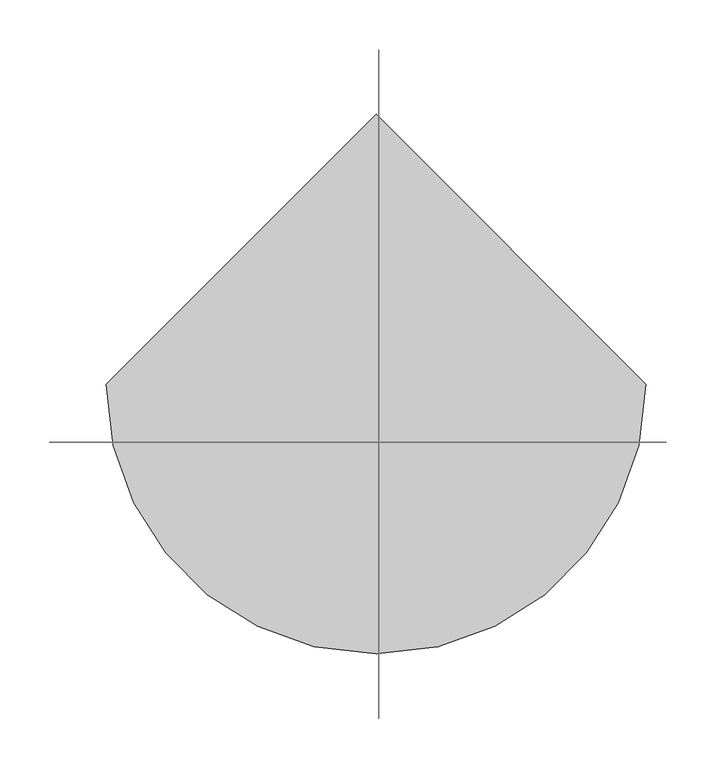
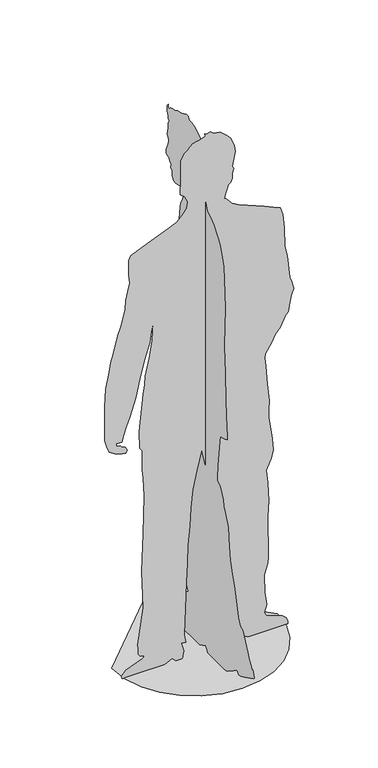
"""IFC4 building model written with IfcOpenShell, lengths in millimetres: proxy geometry, brennan 23759 : brennan 23759."""

from ifc_helpers import new_model, si_unit, origin, place, context, project, spatial, triangles, source, transform, mapped, element, save


def entourage_5001038d(model_context):
    return source(origin(), model_context, "Body", "Tessellation", [
        triangles([(-272.8237541, 0.0, 0.0), (-265.6179985, -62.508739, 0.0), (-245.0759747, -119.914065, 0.0), (-212.8506706, -170.5790321, 0.0), (-170.5790321, -212.8506706, 0.0), (-119.914065, -245.0759747, 0.0), (-62.508739, -265.6179985, 0.0), (0.0, -272.8237541, 0.0), (62.508739, -265.6179985, 0.0), (119.914065, -245.0759747, 0.0), (170.5790321, -212.8506706, 0.0), (212.8506706, -170.5790321, 0.0), (245.0759747, -119.914065, 0.0), (265.6179985, -62.508739, 0.0), (272.8237541, 0.0, 0.0), (0.0, 272.8237541, 0.0), (17.3323325, -58.9941234, 1803.4452976), (28.5662524, -58.9941234, 1794.2976002), (51.3711104, -58.9941234, 1790.7991219), (70.6934502, -58.9941234, 1773.5309898), (84.1902009, -58.9941234, 1758.6380035), (96.7561399, -58.9941234, 1728.4508926), (100.5435813, -58.9941234, 1706.8495949), (90.8824069, -58.9941234, 1658.3351143), (94.6698392, -58.9941234, 1649.7491558), (90.8824069, -58.9941234, 1634.1179878), (91.1873301, -58.9941234, 1616.5128124), (85.8271467, -58.9941234, 1604.5888309), (77.5300878, -58.9941234, 1597.8966522), (73.501927, -58.9941234, 1586.9836555), (68.8960218, -58.9941234, 1573.3586151), (64.8036662, -58.9941234, 1555.3682888), (71.4316773, -58.9941234, 1551.0351231), (89.1331223, -58.9941234, 1530.3004875), (111.1516093, -58.9941234, 1515.9371201), (196.7219676, -58.9941234, 1481.0959328), (225.657338, -58.9941234, 1468.1127136), (247.9325954, -58.9941234, 1457.5047855), (256.0691627, -58.9941234, 1432.3247818), (262.215717, -58.9941234, 1382.7991711), (262.66509, -58.9941234, 1321.2533638), (271.5880192, -58.9941234, 1282.6247623), (279.4517653, -58.9941234, 1205.6402899), (284.9242873, -58.9941234, 1193.4594927), (293.4941676, -58.9941234, 1162.1650366), (284.2181531, -58.9941234, 1141.3180532), (280.6072543, -58.9941234, 1114.9985842), (275.7927226, -58.9941234, 1086.5607124), (264.7353307, -58.9941234, 1075.5033205), (249.1201864, -58.9941234, 1041.994174), (232.4458408, -58.9941234, 1023.1532455), (220.2169179, -58.9941234, 999.2892225), (205.9658801, -58.9941234, 976.5806522), (198.7601244, -58.9941234, 964.9294739), (196.7701296, -58.9941234, 951.8820871), (200.0600633, -58.9941234, 923.7972462), (205.0190266, -58.9941234, 860.4700796), (212.3050281, -58.9941234, 798.3625334), (211.149539, -58.9941234, 769.7963264), (210.4273629, -58.9941234, 741.8559534), (222.8488612, -58.9941234, 662.8173185), (225.7375839, -58.9941234, 622.9850115), (219.783605, -58.9941234, 595.2853941), (202.3710232, -58.9941234, 560.3639428), (207.8917073, -58.9941234, 513.5987377), (210.2187274, -58.9941234, 450.4159664), (207.9398512, -58.9941234, 397.7288844), (208.9027466, -58.9941234, 255.6840118), (207.233717, -58.9941234, 233.2482628), (195.7751141, -58.9941234, 197.7330251), (197.8774567, -58.9941234, 134.2774325), (204.9387807, -58.9941234, 92.0539469), (196.6417399, -58.9941234, 65.5739907), (202.0179743, -58.9941234, 54.6289466), (255.0581052, -58.9941234, 33.717807), (267.6721972, -58.9941234, 23.7196187), (272.9039999, -58.9941234, 10.2549632), (273.241007, -58.9941234, 0.6900836), (261.9268538, -58.9941234, 0.0), (221.8699057, -58.9941234, 0.0), (191.6025126, -58.9941234, 0.0), (171.4616999, -58.9941234, 0.0), (142.0127888, -58.9941234, 0.0), (122.658347, -58.9941234, 10.2549632), (115.8538023, -58.9941234, 0.0), (84.7037506, -58.9941234, 0.0), (81.3977659, -58.9941234, 24.6504281), (90.4972469, -58.9941234, 46.3800406), (91.4601514, -58.9941234, 126.9111943), (80.8842163, -58.9941234, 157.4835015), (66.3122224, -58.9941234, 219.2861063), (39.8483172, -58.9941234, 475.5318026), (27.828023, -58.9941234, 536.9973822), (20.5099263, -58.9941234, 568.3079347), (16.1768435, -58.9941234, 596.7939503), (7.3020474, -58.9941234, 627.8958309), (0.1283877, -58.9941234, 657.1200645), (-6.290995, -58.9941234, 688.2861855), (-10.7524653, -58.9941234, 704.8000757), (-18.1668519, -58.9941234, 671.7563078), (-27.0095523, -58.9941234, 638.4076166), (-40.0408972, -58.9941234, 577.9049143), (-46.7170567, -58.9941234, 516.1504352), (-49.7181181, -58.9941234, 452.6627406), (-56.8436324, -58.9941234, 389.7046649), (-58.3682351, -58.9941234, 326.3132581), (-60.7113106, -58.9941234, 262.1675732), (-67.9652101, -58.9941234, 81.9755105), (-63.4555971, -58.9941234, 53.5857962), (-78.1720272, -58.9941234, 56.1374982), (-69.4416689, -58.9941234, 26.5441465), (-73.501927, -58.9941234, 0.0), (-95.0389573, -58.9941234, 0.0), (-107.8616757, -58.9941234, 13.0634434), (-134.0688061, -58.9941234, 0.0), (-208.1805705, -58.9941234, 0.0), (-272.502789, -58.9941234, 0.0), (-275.9692562, -58.9941234, 8.0402767), (-260.4503996, -58.9941234, 25.870112), (-206.5115408, -58.9941234, 46.4602818), (-198.5033632, -58.9941234, 54.3079769), (-212.6741371, -58.9941234, 57.3892795), (-219.1737585, -58.9941234, 67.1788392), (-219.815707, -58.9941234, 83.0026189), (-221.1316695, -58.9941234, 100.3991406), (-203.3339368, -58.9941234, 222.7365316), (-207.570724, -58.9941234, 352.2636), (-203.2216072, -58.9941234, 481.1808764), (-199.5946484, -58.9941234, 609.8252769), (-202.3068375, -58.9941234, 673.7944101), (-205.3079079, -58.9941234, 703.8050783), (-205.3079079, -58.9941234, 732.3552252), (-205.3399917, -58.9941234, 770.3258726), (-213.9259139, -58.9941234, 781.5919001), (-215.4023862, -58.9941234, 839.8317318), (-202.5636168, -58.9941234, 966.2615147), (-197.1392386, -58.9941234, 997.1868799), (-195.4220469, -58.9941234, 1026.4432337), (-183.626437, -58.9941234, 1084.4583698), (-173.2751793, -58.9941234, 1144.7042564), (-170.5790321, -58.9941234, 1206.314304), (-177.1910013, -58.9941234, 1174.9877277), (-181.6524841, -58.9941234, 1138.0923054), (-199.6267503, -58.9941234, 1082.6448904), (-213.5568048, -58.9941234, 1022.9606701), (-228.0325201, -58.9941234, 962.1691772), (-247.0980715, -58.9941234, 902.2602613), (-258.3962009, -58.9941234, 872.7632246), (-267.6882573, -58.9941234, 847.5992083), (-272.839796, -58.9941234, 824.0240484), (-292.2744927, -58.9941234, 824.489427), (-290.9424701, -58.9941234, 815.7911934), (-278.2320904, -58.9941234, 813.1271118), (-273.5459302, -58.9941234, 807.1089472), (-261.8305661, -58.9941234, 802.7758541), (-256.2456963, -58.9941234, 789.6161196), (-260.1775784, -58.9941234, 781.6881878), (-271.3472999, -58.9941234, 782.6992453), (-291.2634353, -58.9941234, 788.7174099), (-315.0151468, -58.9941234, 803.7548641), (-321.4024386, -58.9941234, 818.9687611), (-329.057531, -58.9941234, 849.2361723), (-330.3895718, -58.9941234, 967.3527998), (-325.7836756, -58.9941234, 1027.5986864), (-315.1274946, -58.9941234, 1082.5807228), (-309.9277757, -58.9941234, 1113.490028), (-301.9035562, -58.9941234, 1140.2909357), (-287.010588, -58.9941234, 1198.739403), (-277.2049911, -58.9941234, 1225.7650063), (-261.509601, -58.9941234, 1282.5445347), (-260.5145854, -58.9941234, 1311.6564205), (-254.4322168, -58.9941234, 1341.3139126), (-246.8894541, -58.9941234, 1367.6333817), (-249.7942187, -58.9941234, 1397.5798096), (-250.1472858, -58.9941234, 1447.3620907), (-243.5192747, -58.9941234, 1462.4637852), (-188.2644351, -58.9941234, 1487.1622776), (-118.1166366, -58.9941234, 1514.0915932), (-91.7329727, -58.9941234, 1526.2723904), (-74.1920148, -58.9941234, 1544.6157475), (-58.9138822, -58.9941234, 1564.1628101), (-56.4263705, -58.9941234, 1585.6516148), (-65.2369746, -58.9941234, 1605.9208717), (-80.226235, -58.9941234, 1619.2090141), (-79.9052608, -58.9941234, 1674.7527168), (-79.1509827, -58.9941234, 1735.6726902), (-66.0233501, -58.9941234, 1758.3009602), (-56.3621802, -58.9941234, 1765.3301823), (-49.8144058, -58.9941234, 1773.3384144), (-43.5234153, -58.9941234, 1777.3665115), (-39.1261365, -58.9941234, 1781.3305138), (-27.9564104, -58.9941234, 1785.4388386), (-15.6151477, -58.9941234, 1787.6215542), (1.7492817, -58.9941234, 1793.366843), (-0.7221805, -58.9941234, 1802.7712109), (5.8416379, -58.9941234, 1798.4541779), (2.5035593, 141.7399675, 1771.3162994), (2.5035593, 151.770251, 1759.9539116), (2.5035593, 154.113322, 1767.6251003), (2.5035593, 153.4713917, 1775.9542431), (2.5035593, 158.3822112, 1768.6522179), (2.5035593, 160.5166557, 1751.4803009), (2.5035593, 163.8547332, 1747.6607666), (2.5035593, 157.1143925, 1743.2313858), (2.5035593, 154.0491363, 1734.3887569), (2.5035593, 153.776315, 1724.5028778), (2.5035593, 149.3790271, 1720.4586479), (2.5035593, 153.6800091, 1709.6098915), (2.5035593, 155.1083376, 1690.3998722), (2.5035593, 158.9599557, 1670.0986404), (2.5035593, 151.9307336, 1655.4463371), (2.5035593, 151.6579123, 1645.4642429), (2.5035593, 155.6539802, 1631.3415585), (2.5035593, 161.7202887, 1620.2361317), (2.5035593, 166.4224907, 1609.0341991), (2.5035593, 166.4064488, 1598.7952892), (2.5035593, 159.7944796, 1594.1092381), (2.5035593, 147.7581322, 1592.1031105), (2.5035593, 145.479256, 1581.3507145), (2.5035593, 137.4710784, 1575.7978558), (2.5035593, 138.8191429, 1565.2380352), (2.5035593, 131.0356427, 1557.3421509), (2.5035593, 131.7738698, 1540.6838654), (2.5035593, 121.4386722, 1529.0488197), (2.5035593, 112.8045971, 1527.6204185), (2.5035593, 84.8963351, 1531.9214642), (2.5035593, 77.3054104, 1525.694664), (2.5035593, 65.5097959, 1511.202816), (2.5035593, 72.0254728, 1496.8074738), (2.5035593, 82.0878492, 1476.0567055), (2.5035593, 86.6456106, 1459.8959187), (2.5035593, 90.6898223, 1412.745599), (2.5035593, 98.4091367, 1392.1714188), (2.5035593, 112.4836319, 1350.3492622), (2.5035593, 129.2703162, 1284.6949848), (2.5035593, 131.5331505, 1264.8911064), (2.5035593, 130.136933, 1219.0728275), (2.5035593, 129.5752395, 1177.0418901), (2.5035593, 133.0416976, 1160.1429216), (2.5035593, 147.5655567, 1155.2480896), (2.5035593, 165.2670017, 1146.2449327), (2.5035593, 184.1399776, 1133.999968), (2.5035593, 254.1754556, 1088.6310076), (2.5035593, 271.7164089, 1078.2636898), (2.5035593, 304.8564646, 1064.0447176), (2.5035593, 322.7184194, 1052.0244484), (2.5035593, 330.357488, 1036.3451002), (2.5035593, 338.2693597, 1017.1832611), (2.5035593, 336.6003119, 987.9269073), (2.5035593, 327.5489748, 980.0150356), (2.5035593, 319.6050193, 980.9298054), (2.5035593, 316.122492, 975.9386856), (2.5035593, 297.6186251, 970.4822599), (2.5035593, 287.6685784, 968.2193893), (2.5035593, 278.2962762, 974.0931587), (2.5035593, 276.6914323, 986.9640301), (2.5035593, 249.8744645, 1003.4778477), (2.5035593, 238.4800655, 990.5428087), (2.5035593, 229.0917033, 978.9237505), (2.5035593, 217.4726269, 986.1775955), (2.5035593, 202.2747355, 997.8127865), (2.5035593, 170.2099231, 1016.6857624), (2.5035593, 138.40189, 1032.4132181), (2.5035593, 139.3326926, 1010.6194176), (2.5035593, 140.2635042, 987.7343319), (2.5035593, 144.4040128, 943.0715057), (2.5035593, 152.6689698, 851.2261671), (2.5035593, 151.770251, 797.5922316), (2.5035593, 142.718923, 782.6350777), (2.5035593, 130.3776614, 775.637903), (2.5035593, 110.3170854, 774.979949), (2.5035593, 109.5949093, 753.8601625), (2.5035593, 109.691197, 730.8627291), (2.5035593, 107.1555415, 638.0064056), (2.5035593, 103.5767356, 545.9684916), (2.5035593, 96.4351748, 454.9095511), (2.5035593, 86.0678661, 335.8620938), (2.5035593, 70.6613528, 246.8092083), (2.5035593, 63.7284184, 203.7351478), (2.5035593, 49.2687587, 165.0423243), (2.5035593, 40.105092, 147.453218), (2.5035593, 49.2045684, 140.6647152), (2.5035593, 57.4855718, 132.4639531), (2.5035593, 59.4916267, 126.2853059), (2.5035593, 69.6663463, 91.7811165), (2.5035593, 82.184146, 81.3014782), (2.5035593, 98.681958, 72.8599922), (2.5035593, 118.8388218, 63.6321307), (2.5035593, 137.6797048, 54.3882182), (2.5035593, 170.274127, 38.9014591), (2.5035593, 173.1628497, 33.2524012), (2.5035593, 179.2291582, 30.9093256), (2.5035593, 179.1810143, 19.8840379), (2.5035593, 167.1767688, 11.6351308), (2.5035593, 147.3890232, 6.0502677), (2.5035593, 114.9229907, 0.2567753), (2.5035593, 35.8522516, 0.2567753), (2.5035593, -2.5998498, 0.2567753), (2.5035593, -24.7627668, 0.2567753), (2.5035593, -58.785497, 17.7335435), (2.5035593, -74.3043535, 0.2567753), (2.5035593, -93.4180624, 0.2567753), (2.5035593, -163.4695823, 0.2567753), (2.5035593, -183.7387666, 5.6169599), (2.5035593, -218.0664315, 27.025601), (2.5035593, -234.5160815, 39.0779926), (2.5035593, -240.0849094, 42.5123624), (2.5035593, -248.7671193, 32.4820744), (2.5035593, -261.0923299, 35.4349919), (2.5035593, -281.9553188, 44.422125), (2.5035593, -298.4210471, 51.8525626), (2.5035593, -335.0275881, 69.9391721), (2.5035593, -338.2693597, 75.1388729), (2.5035593, -334.3695977, 83.5161686), (2.5035593, -327.4687471, 96.9968683), (2.5035593, -322.3332321, 96.6759032), (2.5035593, -319.1716882, 105.0371479), (2.5035593, -309.2858454, 121.5028579), (2.5035593, -300.1863645, 141.6436707), (2.5035593, -271.2349521, 200.6057058), (2.5035593, -257.4653893, 207.0090395), (2.5035593, -245.1401605, 231.2261478), (2.5035593, -226.9412168, 319.0433167), (2.5035593, -210.748328, 359.2767983), (2.5035593, -199.0329457, 400.6978529), (2.5035593, -194.651727, 444.6706412), (2.5035593, -188.9224255, 510.4211337), (2.5035593, -172.0875883, 549.6917381), (2.5035593, -163.6781997, 567.9869514), (2.5035593, -159.2167351, 589.6202966), (2.5035593, -152.187513, 606.5995291), (2.5035593, -141.563434, 622.936904), (2.5035593, -124.4236826, 633.849828), (2.5035593, -125.5952135, 645.8059296), (2.5035593, -129.9122556, 688.751564), (2.5035593, -134.9835667, 734.104537), (2.5035593, -140.4400378, 778.5587276), (2.5035593, -143.120134, 798.3785934), (2.5035593, -155.5576924, 801.4919935), (2.5035593, -172.5048593, 806.2744051), (2.5035593, -183.9153002, 811.7469635), (2.5035593, -183.0968363, 828.1163858), (2.5035593, -181.1710273, 852.0285891), (2.5035593, -177.6243143, 896.4667923), (2.5035593, -175.6503613, 942.1727961), (2.5035593, -170.242025, 1034.4032129), (2.5035593, -165.6682127, 1126.6818827), (2.5035593, -171.445658, 1263.238155), (2.5035593, -169.9692038, 1311.1106689), (2.5035593, -166.5669223, 1360.1709011), (2.5035593, -161.8647202, 1402.5388092), (2.5035593, -148.5766051, 1444.9388374), (2.5035593, -142.1572204, 1462.9451511), (2.5035593, -132.3034705, 1480.084948), (2.5035593, -106.4654582, 1512.8559128), (2.5035593, -89.3577997, 1527.9895821), (2.5035593, -69.2490889, 1540.5876503), (2.5035593, -59.9088886, 1561.9641071), (2.5035593, -52.8475646, 1576.0546715), (2.5035593, -40.1371894, 1576.7287582), (2.5035593, -34.022728, 1594.1894657), (2.5035593, -34.8411986, 1602.1334576), (2.5035593, -38.0669374, 1609.8046463), (2.5035593, -40.6507391, 1617.7646255), (2.5035593, -44.7912431, 1626.1258884), (2.5035593, -52.2377226, 1645.5765907), (2.5035593, -56.6670989, 1688.7790409), (2.5035593, -52.671031, 1723.6363609), (2.5035593, -45.4171315, 1740.4551018), (2.5035593, -40.4100107, 1748.0299301), (2.5035593, -36.5904809, 1756.952932), (2.5035593, -25.2442213, 1771.3162994), (2.5035593, -11.9079543, 1780.4478642), (2.5035593, 2.3591231, 1789.3386005), (2.5035593, 19.6112144, 1792.14715), (2.5035593, 33.0919163, 1792.5001808), (2.5035593, 39.30267, 1802.8193184), (2.5035593, 45.031967, 1803.0280266), (2.5035593, 51.7883678, 1803.1884819), (2.5035593, 64.0012442, 1797.1221371), (2.5035593, 76.278311, 1791.5373035), (2.5035593, 88.3948952, 1787.3807259), (2.5035593, 101.057131, 1784.9253525), (2.5035593, 113.2539519, 1777.559087), (2.5035593, 128.4518433, 1776.1146984)], [[15, 16, 1], [14, 15, 1], [14, 1, 2], [13, 14, 2], [13, 2, 3], [13, 3, 4], [12, 13, 4], [11, 12, 4], [11, 4, 5], [11, 5, 6], [11, 6, 7], [11, 7, 8], [11, 8, 9], [11, 9, 10], [194, 195, 196], [108, 109, 110], [77, 78, 79], [85, 86, 87], [84, 85, 87], [84, 87, 88], [111, 112, 113], [111, 113, 114], [110, 111, 114], [149, 150, 151], [156, 157, 158], [155, 156, 158], [154, 155, 158], [154, 158, 159], [153, 154, 159], [152, 153, 159], [152, 159, 160], [152, 160, 161], [151, 152, 161], [151, 161, 162], [149, 151, 162], [149, 162, 163], [148, 149, 163], [147, 148, 163], [146, 147, 163], [146, 163, 164], [145, 146, 164], [145, 164, 165], [144, 145, 165], [144, 165, 166], [144, 166, 167], [143, 144, 167], [143, 167, 168], [142, 143, 168], [142, 168, 169], [141, 142, 169], [141, 169, 170], [76, 77, 79], [76, 79, 80], [75, 76, 80], [74, 75, 80], [74, 80, 81], [74, 81, 82], [116, 117, 118], [116, 118, 119], [116, 119, 120], [115, 116, 120], [115, 120, 121], [114, 115, 121], [110, 114, 121], [108, 110, 121], [107, 108, 121], [107, 121, 122], [107, 122, 123], [107, 123, 124], [107, 124, 125], [107, 125, 126], [107, 126, 127], [106, 107, 127], [105, 106, 127], [105, 127, 128], [104, 105, 128], [103, 104, 128], [103, 128, 129], [102, 103, 129], [101, 102, 129], [101, 129, 130], [100, 101, 130], [100, 130, 131], [99, 100, 131], [99, 131, 132], [99, 132, 133], [196, 17, 18], [194, 196, 18], [74, 82, 83], [73, 74, 83], [73, 83, 84], [73, 84, 88], [73, 88, 89], [72, 73, 89], [71, 72, 89], [70, 71, 89], [70, 89, 90], [70, 90, 91], [69, 70, 91], [69, 91, 92], [68, 69, 92], [67, 68, 92], [66, 67, 92], [65, 66, 92], [65, 92, 93], [64, 65, 93], [64, 93, 94], [64, 94, 95], [63, 64, 95], [62, 63, 95], [61, 62, 95], [61, 95, 96], [60, 61, 96], [60, 96, 97], [60, 97, 98], [60, 98, 99], [59, 60, 99], [58, 59, 99], [57, 58, 99], [56, 57, 99], [56, 99, 133], [55, 56, 133], [55, 133, 134], [55, 134, 135], [55, 135, 136], [55, 136, 137], [54, 55, 137], [54, 137, 138], [54, 138, 139], [54, 139, 140], [53, 54, 140], [52, 53, 140], [51, 52, 140], [51, 140, 141], [50, 51, 141], [49, 50, 141], [48, 49, 141], [47, 48, 141], [46, 47, 141], [45, 46, 141], [44, 45, 141], [43, 44, 141], [42, 43, 141], [41, 42, 141], [40, 41, 141], [39, 40, 141], [38, 39, 141], [37, 38, 141], [36, 37, 141], [35, 36, 141], [34, 35, 141], [34, 141, 170], [34, 170, 171], [34, 171, 172], [34, 172, 173], [34, 173, 174], [34, 174, 175], [34, 175, 176], [34, 176, 177], [34, 177, 178], [34, 178, 179], [34, 179, 180], [33, 34, 180], [32, 33, 180], [32, 180, 181], [32, 181, 182], [31, 32, 182], [30, 31, 182], [29, 30, 182], [29, 182, 183], [183, 184, 185], [29, 183, 185], [28, 29, 185], [27, 28, 185], [26, 27, 185], [25, 26, 185], [24, 25, 185], [24, 185, 186], [23, 24, 186], [23, 186, 187], [23, 187, 188], [22, 23, 188], [21, 22, 188], [20, 21, 188], [19, 20, 188], [18, 19, 188], [194, 18, 188], [193, 194, 188], [192, 193, 188], [191, 192, 188], [190, 191, 188], [190, 188, 189], [199, 200, 201], [202, 203, 204], [199, 201, 202], [198, 199, 202], [258, 259, 260], [291, 292, 293], [291, 293, 294], [198, 202, 204], [340, 341, 342], [314, 315, 316], [307, 308, 309], [358, 359, 360], [291, 294, 295], [290, 291, 295], [289, 290, 295], [289, 295, 296], [288, 289, 296], [288, 296, 297], [287, 288, 297], [286, 287, 297], [285, 286, 297], [285, 297, 298], [376, 377, 378], [312, 313, 314], [311, 312, 314], [311, 314, 316], [284, 285, 298], [284, 298, 299], [284, 299, 300], [283, 284, 300], [282, 283, 300], [281, 282, 300], [215, 216, 217], [215, 217, 218], [214, 215, 218], [213, 214, 218], [220, 221, 222], [254, 255, 256], [253, 254, 256], [252, 253, 256], [251, 252, 256], [258, 260, 261], [257, 258, 261], [311, 316, 317], [311, 317, 318], [310, 311, 318], [339, 340, 342], [339, 342, 343], [338, 339, 343], [300, 301, 302], [249, 250, 251], [248, 249, 251], [248, 251, 256], [247, 248, 256], [247, 256, 257], [246, 247, 257], [245, 246, 257], [244, 245, 257], [243, 244, 257], [243, 257, 261], [243, 261, 262], [242, 243, 262], [242, 262, 263], [241, 242, 263], [240, 241, 263], [239, 240, 263], [309, 310, 318], [307, 309, 318], [307, 318, 319], [307, 319, 320], [307, 320, 321], [306, 307, 321], [305, 306, 321], [205, 206, 207], [304, 305, 321], [303, 304, 321], [302, 303, 321], [300, 302, 321], [281, 300, 321], [281, 321, 322], [281, 322, 323], [280, 281, 323], [279, 280, 323], [278, 279, 323], [278, 323, 324], [277, 278, 324], [277, 324, 325], [276, 277, 325], [276, 325, 326], [276, 326, 327], [276, 327, 328], [275, 276, 328], [275, 328, 329], [275, 329, 330], [275, 330, 331], [275, 331, 332], [275, 332, 333], [274, 275, 333], [273, 274, 333], [273, 333, 334], [273, 334, 335], [273, 335, 336], [272, 273, 336], [272, 336, 337], [271, 272, 337], [271, 337, 338], [271, 338, 343], [271, 343, 344], [271, 344, 345], [271, 345, 346], [271, 346, 347], [270, 271, 347], [269, 270, 347], [268, 269, 347], [267, 268, 347], [266, 267, 347], [265, 266, 347], [264, 265, 347], [263, 264, 347], [239, 263, 347], [238, 239, 347], [238, 347, 348], [237, 238, 348], [236, 237, 348], [235, 236, 348], [234, 235, 348], [234, 348, 349], [234, 349, 350], [233, 234, 350], [232, 233, 350], [232, 350, 351], [232, 351, 352], [231, 232, 352], [231, 352, 353], [231, 353, 354], [231, 354, 355], [231, 355, 356], [230, 231, 356], [229, 230, 356], [229, 356, 357], [228, 229, 357], [228, 357, 358], [228, 358, 360], [227, 228, 360], [227, 360, 361], [226, 227, 361], [226, 361, 362], [222, 223, 224], [222, 224, 225], [222, 225, 226], [222, 226, 362], [220, 222, 362], [220, 362, 363], [220, 363, 364], [220, 364, 365], [220, 365, 366], [220, 366, 367], [220, 367, 368], [220, 368, 369], [220, 369, 370], [219, 220, 370], [218, 219, 370], [213, 218, 370], [212, 213, 370], [211, 212, 370], [210, 211, 370], [209, 210, 370], [208, 209, 370], [207, 208, 370], [207, 370, 371], [207, 371, 372], [207, 372, 373], [207, 373, 374], [207, 374, 375], [207, 375, 376], [207, 376, 378], [207, 378, 379], [207, 379, 380], [207, 380, 381], [207, 381, 382], [207, 382, 383], [207, 383, 384], [205, 207, 384], [205, 384, 385], [205, 385, 197], [205, 197, 198], [205, 198, 204]], closed=False),
    ])


if __name__ == "__main__":
    model = new_model("IFC4")
    model_context = context("Model", 3, world=origin())
    ifc_project = project(units=[si_unit("LENGTHUNIT", "METRE", prefix="MILLI")], contexts=[model_context])
    site = spatial("IfcSite", under=ifc_project)
    building = spatial("IfcBuilding", under=site)
    placement = place(None, origin())
    entourage_shape = entourage_5001038d(model_context)
    element("IfcBuildingElementProxy", 1, Name="brennan 23759 : brennan 23759", ObjectType="brennan 23759 : brennan 23759", at=placement, inside=building, context=model_context, shape_type="MappedRepresentation", body=[
        mapped(entourage_shape, transform((0.0, 0.0, 0.0), x_axis=(1.0, 0.0, 0.0), y_axis=(0.0, 1.0, 0.0), z_axis=(0.0, 0.0, 1.0))),
    ])
    save(model, "model.ifc")

# Revit data of these elements
# Type "brennan 23759 : brennan 23759"
#   built-in parameter 1005195 = "RPC-16-64WN-ANPL-8FT0-ALHV-R9RA-Q12N-54"
#   Height = 0
